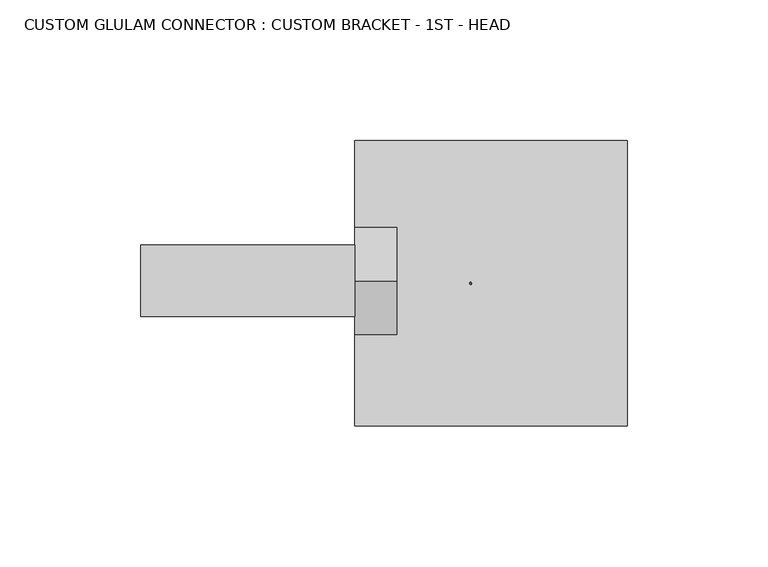
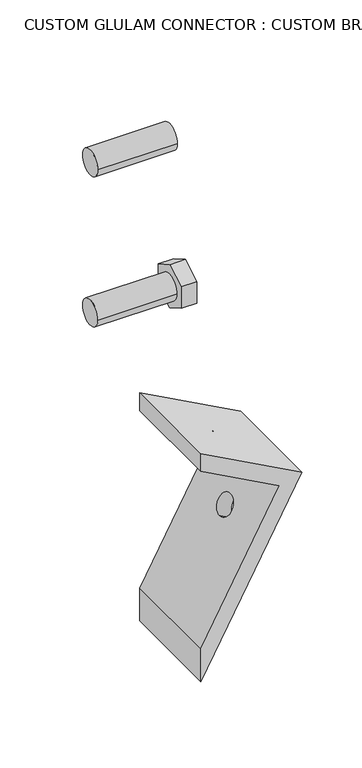
"""IFC4 building model written with IfcOpenShell, lengths in millimetres: fastener geometry, CUSTOM GLULAM CONNECTOR : CUSTOM BRACKET - 1ST - HEAD."""

from ifc_helpers import new_model, si_unit, point, frame, frame_2d, origin, place, context, project, spatial, polyline, circle_curve, trimmed, segment, composite_curve, outline, extrude, source, transform, mapped, element, save
from ifc_brep_helpers import plane_surface, revolved_surface, advanced_brep


def custom_glulam_connector_custom_bracket_1st_head_121296cc(model_context):
    return source(origin(), model_context, "Body", "SolidModel", [
        extrude(outline(composite_curve([segment(trimmed(circle_curve(frame_2d((0.79375, 566.7375)), 12.7), [point((-11.90625, 566.7375))], [point((13.49375, 566.7375))], False, "CARTESIAN"), True, "CONTINUOUS"), segment(trimmed(circle_curve(frame_2d((0.79375, 566.7375)), 12.7), [point((13.49375, 566.7375))], [point((-11.90625, 566.7375))], False, "CARTESIAN"), True, "CONTINUOUS")], self_intersect=False)), frame((19.05, 0.0, 0.0), z_axis=(1.0, 0.0, 0.0), x_axis=(0.0, 1.0, 0.0)), (0.0, 0.0, 1.0), 76.2),
        extrude(outline(polyline([(-18.25625, 425.3360226), (0.79375, 436.3345453), (19.84375, 425.3360226), (19.84375, 403.3389774), (0.79375, 392.3404547), (-18.25625, 403.3389774), (-18.25625, 425.3360226)])), frame((95.25, 0.0, 0.0), z_axis=(1.0, 0.0, 0.0), x_axis=(0.0, 1.0, 0.0)), (0.0, 0.0, 1.0), 14.9820312),
        extrude(outline(composite_curve([segment(trimmed(circle_curve(frame_2d((0.79375, 414.3375)), 12.7), [point((-11.90625, 414.3375))], [point((13.49375, 414.3375))], False, "CARTESIAN"), True, "CONTINUOUS"), segment(trimmed(circle_curve(frame_2d((0.79375, 414.3375)), 12.7), [point((13.49375, 414.3375))], [point((-11.90625, 414.3375))], False, "CARTESIAN"), True, "CONTINUOUS")], self_intersect=False)), frame((19.05, 0.0, 0.0), z_axis=(1.0, 0.0, 0.0), x_axis=(0.0, 1.0, 0.0)), (0.0, 0.0, 1.0), 76.2),
        advanced_brep(
        [(192.2086601, -50.8, 223.0256373), (95.25, -50.8, 275.6698944), (95.25, -50.8, 257.6058402), (170.6825431, -50.8, 216.6493109), (95.25, -50.8, 77.7198492), (95.25, -50.8, 44.45), (192.2086601, 50.8, 223.0256373), (95.25, 50.8, 44.45), (95.25, 50.8, 77.7198492), (170.6825431, 50.8, 216.6493109), (95.25, 50.8, 257.6058402), (95.25, 50.8, 275.6698944), (136.752554, 0.0, 253.1358462), (136.0549929, 0.0, 253.514591), (128.4800976, 0.0, 239.5633693), (129.1776587, 0.0, 239.1846245), (153.0709115, 0.0, 184.2127206), (142.8448028, 0.0, 165.3785713), (156.7960245, 0.0, 157.803676), (167.0221331, 0.0, 176.6378253)],
        [
            (0, 1),
            (1, 2),
            (2, 3),
            (3, 4),
            (4, 5),
            (5, 0),
            (6, 7),
            (7, 8),
            (8, 9),
            (9, 10),
            (10, 11),
            (11, 6),
            (0, 6),
            (11, 1),
            (12, 13, circle_curve(frame((136.4037734, 0.0, 253.3252186), z_axis=(-0.47715876025961074, 0.0, -0.8788171126619642), x_axis=(-0.8788171126619642, 0.0, 0.47715876025961074)), 0.396875)),
            (13, 12, circle_curve(frame((136.4037734, 0.0, 253.3252186), z_axis=(-0.47715876025961074, 0.0, -0.8788171126619642), x_axis=(-0.8788171126619642, 0.0, 0.47715876025961074)), 0.396875)),
            (10, 2),
            (9, 3),
            (14, 15, circle_curve(frame((128.8288781, 0.0, 239.3739969), z_axis=(0.47715876025961074, 0.0, 0.8788171126619642), x_axis=(-0.8788171126619642, 0.0, 0.47715876025961074)), 0.396875)),
            (15, 14, circle_curve(frame((128.8288781, 0.0, 239.3739969), z_axis=(0.47715876025961074, 0.0, 0.8788171126619642), x_axis=(-0.8788171126619642, 0.0, 0.47715876025961074)), 0.396875)),
            (8, 4),
            (16, 17, circle_curve(frame((147.9578571, 0.0, 174.795646), z_axis=(0.8788171126619635, 0.0, -0.47715876025961207), x_axis=(0.47715876025961207, 0.0, 0.8788171126619635)), 10.715625)),
            (17, 16, circle_curve(frame((147.9578571, 0.0, 174.795646), z_axis=(0.8788171126619635, 0.0, -0.47715876025961207), x_axis=(0.47715876025961207, 0.0, 0.8788171126619635)), 10.715625)),
            (7, 5),
            (18, 19, circle_curve(frame((161.9090788, 0.0, 167.2207506), z_axis=(-0.8788171126619635, 0.0, 0.47715876025961207), x_axis=(0.47715876025961207, 0.0, 0.8788171126619635)), 10.715625)),
            (19, 18, circle_curve(frame((161.9090788, 0.0, 167.2207506), z_axis=(-0.8788171126619635, 0.0, 0.47715876025961207), x_axis=(0.47715876025961207, 0.0, 0.8788171126619635)), 10.715625)),
            (12, 15),
            (14, 13),
            (18, 17),
            (16, 19),
        ],
        [
            plane_surface(frame((95.25, -50.8, 275.6698944), z_axis=(0.0, -1.0, 0.0), x_axis=(-0.8788171126619642, 0.0, 0.47715876025961074))),
            plane_surface(frame((95.25, 50.8, 275.6698944), z_axis=(0.0, 1.0, 0.0), x_axis=(0.8788171126619642, 0.0, -0.47715876025961074))),
            plane_surface(frame((192.2086601, -50.8, 223.0256373), z_axis=(0.47715876025961074, 0.0, 0.8788171126619642), x_axis=(0.0, 1.0, 0.0))),
            plane_surface(frame((95.25, -50.8, 275.6698944), z_axis=(-1.0, 0.0, 0.0), x_axis=(0.0, 1.0, 0.0))),
            plane_surface(frame((95.25, -50.8, 257.6058402), z_axis=(-0.4771587602596111, 0.0, -0.8788171126619639), x_axis=(0.0, 1.0, 0.0))),
            plane_surface(frame((170.6825431, -50.8, 216.6493109), z_axis=(-0.8788171126619635, 0.0, 0.477158760259612), x_axis=(0.0, 1.0, 0.0))),
            plane_surface(frame((95.25, -50.8, 77.7198492), z_axis=(-1.0, 0.0, 0.0), x_axis=(0.0, 1.0, 0.0))),
            plane_surface(frame((95.25, -50.8, 44.45), z_axis=(0.8788171126619635, 0.0, -0.47715876025961207), x_axis=(0.0, 1.0, 0.0))),
            revolved_surface(polyline([(128.4800975283424, 0.0, 239.56336929930464), (136.0549928750189, 0.0, 253.51459101356363)]), (136.4037734, 0.0, 253.3252186), (-0.47715876025961074, 0.0, -0.8788171126619642)),
            revolved_surface(polyline([(153.0709114148, 0.0, 184.21272057570627), (167.02213316202443, 0.0, 176.63782521113097)]), (161.9090788, 0.0, 167.2207506), (-0.8788171126619635, 0.0, 0.47715876025961207)),
        ],
        [
            (0, [[1, 2, 3, 4, 5, 6]]),
            (1, [[7, 8, 9, 10, 11, 12]]),
            (2, [[-1, 13, -12, 14], [15, 16]]),
            (3, [[-2, -14, -11, 17]]),
            (4, [[-3, -17, -10, 18], [19, 20]]),
            (5, [[-4, -18, -9, 21], [22, 23]]),
            (6, [[-5, -21, -8, 24]]),
            (7, [[-6, -24, -7, -13], [25, 26]]),
            (8, [[27, -19, 28, -15]]),
            (8, [[-27, -16, -28, -20]]),
            (9, [[29, -22, 30, -25]]),
            (9, [[-29, -26, -30, -23]]),
        ],
    ),
    ])


if __name__ == "__main__":
    model = new_model("IFC4")
    model_context = context("Model", 3, world=origin())
    ifc_project = project(units=[si_unit("LENGTHUNIT", "METRE", prefix="MILLI")], contexts=[model_context])
    site = spatial("IfcSite", under=ifc_project)
    building = spatial("IfcBuilding", under=site)
    placement = place(None, origin())
    custom_glulam_connector_custom_bracket_1st_head_shape = custom_glulam_connector_custom_bracket_1st_head_121296cc(model_context)
    element("IfcFastener", 1, ObjectType="CUSTOM GLULAM CONNECTOR : CUSTOM BRACKET - 1ST - HEAD", at=placement, inside=building, context=model_context, shape_type="MappedRepresentation", body=[
        mapped(custom_glulam_connector_custom_bracket_1st_head_shape, transform((0.0, 0.0, 0.0), x_axis=(1.0, 0.0, 0.0), y_axis=(0.0, 1.0, 0.0), z_axis=(0.0, 0.0, 1.0))),
    ])
    save(model, "model.ifc")

# Revit data of these elements
# Type "CUSTOM GLULAM CONNECTOR : CUSTOM BRACKET - 1ST - HEAD"
#   Width - Top = 0' - 6 7/8"
#   Top/Bottom Plate Thickness = 0' - 0 5/16"
#   Top/Bottom Plate - Width = 0' - 7 1/2"
#   Rod Radius = 0' - 0 3/8"
#   Rod Length [instance default] = 1' - 0"
#   Plate Thickness = 0' - 0 5/16"
#   Offset - Upper Plate 2 = 0' - 1"
#   Height of Plate = 1' - 1"
#   Width - Bottom = 0' - 6 7/8"
#   Plate Width = 0' - 4 3/4"
#   Bracket Width = 0' - 4"
#   Bracket Thickness = 0' - 0 5/8"
#   Bracket Offset in X = 0' - 3 3/4"
#   Bracket Offset in Y = 0' - 0 3/8"
#   Bracket Offset = 0' - 1 3/4"
#   Bracket Leg = 0' - 8"
#   Bracket Hole Radius - Up = 0' - 0 1/64"
#   Bracket Hole Radius - Down = 0' - 0 27/64"
#   Bracket Hole Offset = 0' - 2 1/2"
#   Beam Width = 0' - 7 3/8"
#   Angle 2 = 61.50°
#   Angle 1 = 151.50°
#   Top Plate Visible = no
#   Rod Visibility = no
#   Plate Visibility - Upper Right 2 = yes
#   Plate Visibility - Upper Right 1 = yes
#   Plate Visibility - Upper Left 2 = yes
#   Plate Visibility - Upper Left 1 = yes
#   Plate Visibility - Lower Right 2 = no
#   Plate Visibility - Lower Right 1 = yes
#   Plate Visibility - Lower Left 2 = no
#   Plate Visibility - Lower Left 1 = yes
#   Bracket Visibility = yes
#   Bottom Plate Visible = no
#   Upper Plates - 2 = element 1119951
#   Upper Plates - 1 = element 1951456
#   Lower Plates = element 1135840
#   Bracket Material = 5/8" STEEL ANGLE (HDG AFTER FABRICATION)
#   URL = ""
# Element 1 (IfcFastener, "CUSTOM GLULAM CONNECTOR : CUSTOM BRACKET - 1ST - HEAD")
#   Materials on its faces: "1\" GALV. LAG BOLT (LENGTH = 1/2\" SHY OF GLULAM DEPTH) -  (GALV. THRU BOLT IF PLATE ON OPP. SIDE OF STRUCT MEMBER)", "5/16\" STEEL PLATE (HDG AFTER FABRICATION)", "5/8\" STEEL ANGLE (HDG AFTER FABRICATION)"
# Materials
#   "5/8\" STEEL ANGLE (HDG AFTER FABRICATION)": class "Generic", colour RGB 195 195 195, transparency 0, Cost = 0
#   "1\" GALV. LAG BOLT (LENGTH = 1/2\" SHY OF GLULAM DEPTH) -  (GALV. THRU BOLT IF PLATE ON OPP. SIDE OF STRUCT MEMBER)": class "Generic", colour RGB 120 120 120, transparency 0, Cost = 0
#   "5/16\" STEEL PLATE (HDG AFTER FABRICATION)": class "Generic", colour RGB 232 232 232, transparency 0, Cost = 0
